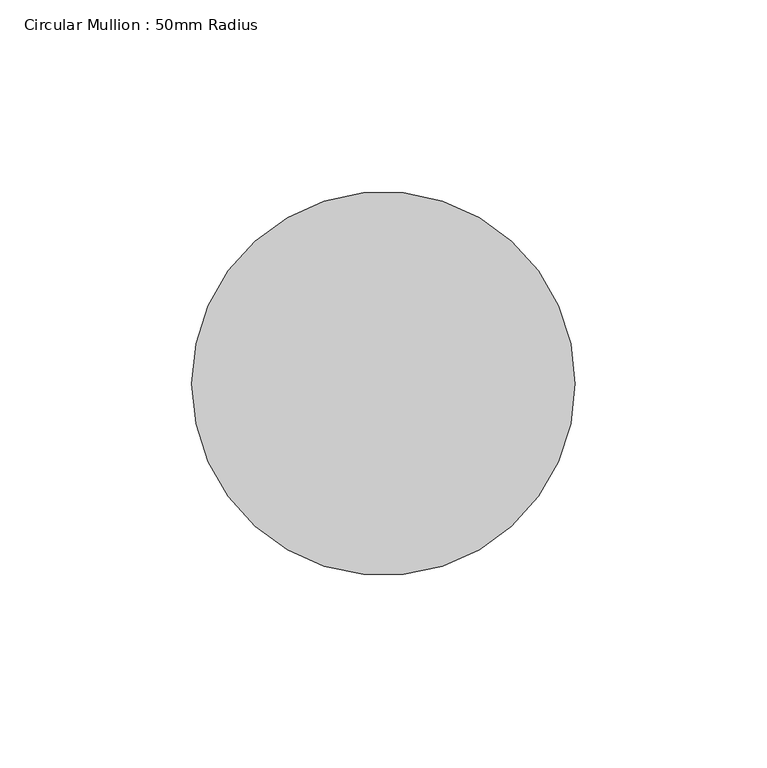
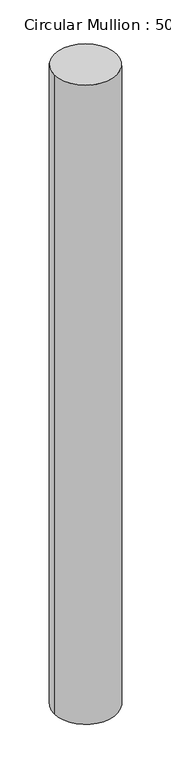
"""IFC4 building model written with IfcOpenShell, lengths in millimetres: member geometry, Circular Mullion : 50mm Radius."""

import ifcopenshell
import ifcopenshell.guid

model = None  # the IFC model being written
_history = None  # IfcOwnerHistory: only IFC2X3 demands one
_inside = {}  # id of a spatial element -> (the spatial element, [elements in it])
_under = {}  # id of a project, library or spatial element -> (it, [spatial elements below it])
_declared = {}  # id of a project -> (the project, [libraries it declares])
_typed = {}  # id of a type object -> (the type object, [elements of that type])
_made_of = {}  # id of a material, layer set ... -> (it, [elements and type objects made of it])


def new_model(schema):
    """Start an empty IFC model of exactly this schema.

    Asked for "IFC4X3", IfcOpenShell would pick the latest addendum, in which some entities
    have other attributes; the version numbers below select the first issue.
    IFC2X3 requires an IfcOwnerHistory on every rooted entity: one is made here for all.
    """
    global model, _history
    if schema == "IFC4X3":
        model = ifcopenshell.file(schema_version=(4, 3, 0, 0))
    else:
        model = ifcopenshell.file(schema=schema)
    _inside.clear()
    _under.clear()
    _declared.clear()
    _typed.clear()
    _made_of.clear()
    _history = None
    if model.schema == "IFC2X3":
        org = make("IfcOrganization", Name="unknown")
        user = make(
            "IfcPersonAndOrganization",
            ThePerson=make("IfcPerson", FamilyName="unknown"),
            TheOrganization=org,
        )
        app = make(
            "IfcApplication",
            ApplicationDeveloper=org,
            Version="unknown",
            ApplicationFullName="unknown",
            ApplicationIdentifier="unknown",
        )
        _history = make(
            "IfcOwnerHistory",
            OwningUser=user,
            OwningApplication=app,
            ChangeAction="ADDED",
            CreationDate=0,
        )
    return model


def make(cls, **values):
    """One entity of the class cls with the attributes given. An attribute that is None is left unset."""
    return model.create_entity(
        cls, **{name: value for name, value in values.items() if value is not None}
    )


def rooted(cls, **values):
    """An entity with a GlobalId (a new one), such as an element, a storey or a relation."""
    return make(cls, GlobalId=ifcopenshell.guid.new(), OwnerHistory=_history, **values)


def si_unit(unit_type, name, prefix=None):
    """IfcSIUnit, for example si_unit("LENGTHUNIT", "METRE", prefix="MILLI")."""
    return make("IfcSIUnit", UnitType=unit_type, Prefix=prefix, Name=name)


def assignment(units):
    """IfcUnitAssignment: the units of a project."""
    return None if units is None else make("IfcUnitAssignment", Units=units)


def point(xyz):
    """IfcCartesianPoint."""
    return None if xyz is None else make("IfcCartesianPoint", Coordinates=xyz)


def direction(xyz):
    """IfcDirection."""
    return None if xyz is None else make("IfcDirection", DirectionRatios=xyz)


def frame(location, z_axis=None, x_axis=None):
    """IfcAxis2Placement3D, a coordinate frame: its origin and axes. An axis left out is left unset."""
    return make(
        "IfcAxis2Placement3D",
        Location=point(location),
        Axis=direction(z_axis),
        RefDirection=direction(x_axis),
    )


def frame_2d(location, x_axis=None):
    """IfcAxis2Placement2D, a coordinate frame in the plane: its origin and x axis."""
    return make(
        "IfcAxis2Placement2D", Location=point(location), RefDirection=direction(x_axis)
    )


def origin():
    """The frame at (0, 0, 0) with its axes left unset."""
    return frame((0.0, 0.0, 0.0))


def origin_2d():
    """The frame at (0, 0) in the plane with its x axis left unset."""
    return frame_2d((0.0, 0.0))


def place(relative_to, where):
    """IfcLocalPlacement: puts the frame where relative to a parent placement (None: the world)."""
    return make(
        "IfcLocalPlacement", PlacementRelTo=relative_to, RelativePlacement=where
    )


def context(
    kind, dimensions, precision=None, world=None, true_north=None, identifier=None
):
    """IfcGeometricRepresentationContext, for example the 3D "Model" context."""
    return make(
        "IfcGeometricRepresentationContext",
        ContextIdentifier=identifier,
        ContextType=kind,
        CoordinateSpaceDimension=dimensions,
        Precision=precision,
        WorldCoordinateSystem=world,
        TrueNorth=true_north,
    )


def project(units=None, contexts=None):
    """IfcProject with its units and contexts."""
    return rooted(
        "IfcProject",
        Name="project",
        RepresentationContexts=contexts,
        UnitsInContext=assignment(units),
    )


def spatial(cls, under=None, at=None, **own):
    """A site, building, storey or space (cls), placed at a placement, below another one or the project."""
    s = rooted(cls, ObjectPlacement=at, **own)
    if under is not None:
        _under.setdefault(under.id(), (under, []))[1].append(s)
    return s


def circle_curve(where, radius):
    """IfcCircle in the frame where."""
    return make("IfcCircle", Position=where, Radius=radius)


def trimmed(basis, trim1, trim2, sense, master):
    """IfcTrimmedCurve: the piece of a basis curve between two trims."""
    return make(
        "IfcTrimmedCurve",
        BasisCurve=basis,
        Trim1=trim1,
        Trim2=trim2,
        SenseAgreement=sense,
        MasterRepresentation=master,
    )


def segment(curve, same_sense, transition):
    """IfcCompositeCurveSegment."""
    return make(
        "IfcCompositeCurveSegment",
        Transition=transition,
        SameSense=same_sense,
        ParentCurve=curve,
    )


def composite_curve(segments, self_intersect=None):
    """IfcCompositeCurve: segments joined end to end."""
    return make("IfcCompositeCurve", Segments=segments, SelfIntersect=self_intersect)


def outline(outer, holes=None, kind="AREA"):
    """IfcArbitraryClosedProfileDef: a profile drawn as a closed curve; with holes, ...WithVoids."""
    if holes is None:
        return make("IfcArbitraryClosedProfileDef", ProfileType=kind, OuterCurve=outer)
    return make(
        "IfcArbitraryProfileDefWithVoids",
        ProfileType=kind,
        OuterCurve=outer,
        InnerCurves=holes,
    )


def extrude(swept, where, along, depth):
    """IfcExtrudedAreaSolid: the profile swept, set in the frame where, extruded along a direction by depth."""
    return make(
        "IfcExtrudedAreaSolid",
        SweptArea=swept,
        Position=where,
        ExtrudedDirection=direction(along),
        Depth=depth,
    )


def shape(context_of_items, identifier, shape_type, items):
    """IfcShapeRepresentation: the items that make up one representation, for example the "Body"."""
    return make(
        "IfcShapeRepresentation",
        ContextOfItems=context_of_items,
        RepresentationIdentifier=identifier,
        RepresentationType=shape_type,
        Items=items,
    )


def source(mapping_origin, context_of_items, identifier, shape_type, items):
    """IfcRepresentationMap: a shape defined once, which mapped items show again and again."""
    return make(
        "IfcRepresentationMap",
        MappingOrigin=mapping_origin,
        MappedRepresentation=shape(context_of_items, identifier, shape_type, items),
    )


def transform(
    local_origin,
    x_axis=None,
    y_axis=None,
    z_axis=None,
    scale=None,
    scale2=None,
    scale3=None,
    uniform=True,
):
    """IfcCartesianTransformationOperator3D, or its non-uniform kind. x_axis, y_axis, z_axis: its Axis1, 2, 3."""
    if uniform:
        return make(
            "IfcCartesianTransformationOperator3D",
            Axis1=direction(x_axis),
            Axis2=direction(y_axis),
            LocalOrigin=point(local_origin),
            Scale=scale,
            Axis3=direction(z_axis),
        )
    return make(
        "IfcCartesianTransformationOperator3DnonUniform",
        Axis1=direction(x_axis),
        Axis2=direction(y_axis),
        LocalOrigin=point(local_origin),
        Scale=scale,
        Axis3=direction(z_axis),
        Scale2=scale2,
        Scale3=scale3,
    )


def mapped(mapping_source, mapping_target):
    """IfcMappedItem: shows the shape of a source again, moved by a transform."""
    return make(
        "IfcMappedItem", MappingSource=mapping_source, MappingTarget=mapping_target
    )


def made_of(thing, what):
    """Note that an element or type object is made of a material, layer set ...; save() writes the relation."""
    if what is not None:
        _made_of.setdefault(what.id(), (what, []))[1].append(thing)
    return thing


def element(
    cls,
    number,
    at=None,
    inside=None,
    cuts=None,
    type_object=None,
    material=None,
    context=None,
    identifier="Body",
    shape_type=None,
    held_by="IfcProductDefinitionShape",
    body=None,
    shapes=None,
    **own,
):
    """One element of the class cls, such as IfcWall. Its Tag is "e" and its number.

    at: its placement. inside: the storey or other place that contains it. cuts: it is an
    opening in that element (IfcRelVoidsElement). A single representation is given by context,
    identifier, shape_type and body (its items); several are given by shapes. held_by: the class
    of the entity that holds the representations. save() writes the other relations.
    """
    e = rooted(cls, Tag="e%d" % number, ObjectPlacement=at, **own)
    if body is not None:
        shapes = [shape(context, identifier, shape_type, body)]
    if shapes is not None:
        e.Representation = make(held_by, Representations=shapes)
    if inside is not None:
        _inside.setdefault(inside.id(), (inside, []))[1].append(e)
    if cuts is not None:
        rooted(
            "IfcRelVoidsElement", RelatingBuildingElement=cuts, RelatedOpeningElement=e
        )
    if type_object is not None:
        _typed.setdefault(type_object.id(), (type_object, []))[1].append(e)
    return made_of(e, material)


def aggregate(whole, parts):
    """IfcRelAggregates: a whole, such as a stair, and the parts it consists of."""
    return rooted("IfcRelAggregates", RelatingObject=whole, RelatedObjects=parts)


def save(model, path):
    """Write the relations noted so far, then the file.

    IfcRelAggregates (storeys below a building ...), IfcRelContainedInSpatialStructure (elements
    in a storey), IfcRelDefinesByType, IfcRelAssociatesMaterial and IfcRelDeclares: one each for
    every whole, place, type object, material and project.
    """
    for whole, parts in _under.values():
        aggregate(whole, parts)
    for where, things in _inside.values():
        rooted(
            "IfcRelContainedInSpatialStructure",
            RelatedElements=things,
            RelatingStructure=where,
        )
    for kind, things in _typed.values():
        rooted("IfcRelDefinesByType", RelatedObjects=things, RelatingType=kind)
    for what, things in _made_of.values():
        rooted("IfcRelAssociatesMaterial", RelatedObjects=things, RelatingMaterial=what)
    for by, libraries in _declared.values():
        rooted("IfcRelDeclares", RelatingContext=by, RelatedDefinitions=libraries)
    model.write(path)


def circular_mullion_50mm_radius_663f154a(model_context):
    return source(origin(), model_context, "Body", "SweptSolid", [
        extrude(outline(composite_curve([segment(trimmed(circle_curve(origin_2d(), 50.0), [point((50.0, 0.0))], [point((-50.0, 0.0))], False, "CARTESIAN"), True, "CONTINUOUS"), segment(trimmed(circle_curve(origin_2d(), 50.0), [point((-50.0, 0.0))], [point((50.0, 0.0))], False, "CARTESIAN"), True, "CONTINUOUS")], self_intersect=False)), frame((0.0, 0.0, -1079.6388144), z_axis=(0.0, 0.0, 1.0), x_axis=(1.0, 0.0, 0.0)), (0.0, 0.0, 1.0), 1079.6388144),
    ])


if __name__ == "__main__":
    model = new_model("IFC4")
    model_context = context("Model", 3, world=origin())
    ifc_project = project(units=[si_unit("LENGTHUNIT", "METRE", prefix="MILLI")], contexts=[model_context])
    site = spatial("IfcSite", under=ifc_project)
    building = spatial("IfcBuilding", under=site)
    placement = place(None, origin())
    circular_mullion_50mm_radius_shape = circular_mullion_50mm_radius_663f154a(model_context)
    element("IfcMember", 1, ObjectType="Circular Mullion : 50mm Radius", at=placement, inside=building, context=model_context, shape_type="MappedRepresentation", body=[
        mapped(circular_mullion_50mm_radius_shape, transform((0.0, 0.0, 0.0), x_axis=(1.0, 0.0, 0.0), y_axis=(0.0, 1.0, 0.0), z_axis=(0.0, 0.0, 1.0))),
    ])
    save(model, "model.ifc")

# Revit data of these elements
# Type "Circular Mullion : 50mm Radius"
#   built-in parameter 1007350 = 0.164042 (stored number, unit not read)
# Element 1 (IfcMember, "Circular Mullion : 50mm Radius")
#   Materials on its faces: "Aluminium"
# Materials
#   "Aluminium": class "Metal", colour RGB 247 247 247, transparency 0, Description = "Aluminium 6061", Cost = 0
